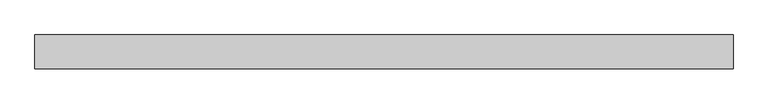
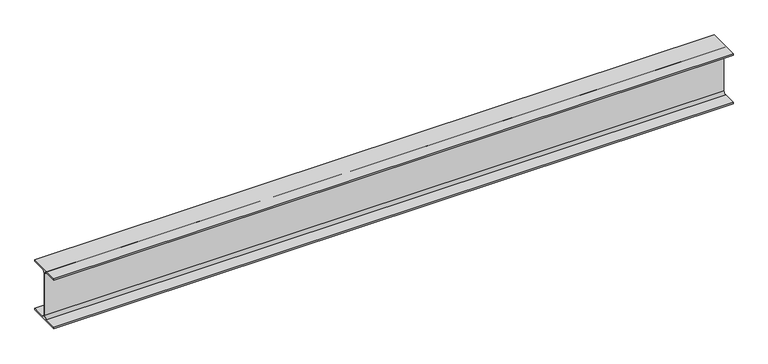
"""IFC4 building model written with IfcOpenShell, lengths in millimetres: beam geometry, 0912_Steel Framing_H-KSD3502 : H_SB_ASB_H-482x300x11x15."""

import ifcopenshell
import ifcopenshell.guid

model = None  # the IFC model being written
_history = None  # IfcOwnerHistory: only IFC2X3 demands one
_inside = {}  # id of a spatial element -> (the spatial element, [elements in it])
_under = {}  # id of a project, library or spatial element -> (it, [spatial elements below it])
_declared = {}  # id of a project -> (the project, [libraries it declares])
_typed = {}  # id of a type object -> (the type object, [elements of that type])
_made_of = {}  # id of a material, layer set ... -> (it, [elements and type objects made of it])


def new_model(schema):
    """Start an empty IFC model of exactly this schema.

    Asked for "IFC4X3", IfcOpenShell would pick the latest addendum, in which some entities
    have other attributes; the version numbers below select the first issue.
    IFC2X3 requires an IfcOwnerHistory on every rooted entity: one is made here for all.
    """
    global model, _history
    if schema == "IFC4X3":
        model = ifcopenshell.file(schema_version=(4, 3, 0, 0))
    else:
        model = ifcopenshell.file(schema=schema)
    _inside.clear()
    _under.clear()
    _declared.clear()
    _typed.clear()
    _made_of.clear()
    _history = None
    if model.schema == "IFC2X3":
        org = make("IfcOrganization", Name="unknown")
        user = make(
            "IfcPersonAndOrganization",
            ThePerson=make("IfcPerson", FamilyName="unknown"),
            TheOrganization=org,
        )
        app = make(
            "IfcApplication",
            ApplicationDeveloper=org,
            Version="unknown",
            ApplicationFullName="unknown",
            ApplicationIdentifier="unknown",
        )
        _history = make(
            "IfcOwnerHistory",
            OwningUser=user,
            OwningApplication=app,
            ChangeAction="ADDED",
            CreationDate=0,
        )
    return model


def make(cls, **values):
    """One entity of the class cls with the attributes given. An attribute that is None is left unset."""
    return model.create_entity(
        cls, **{name: value for name, value in values.items() if value is not None}
    )


def rooted(cls, **values):
    """An entity with a GlobalId (a new one), such as an element, a storey or a relation."""
    return make(cls, GlobalId=ifcopenshell.guid.new(), OwnerHistory=_history, **values)


def si_unit(unit_type, name, prefix=None):
    """IfcSIUnit, for example si_unit("LENGTHUNIT", "METRE", prefix="MILLI")."""
    return make("IfcSIUnit", UnitType=unit_type, Prefix=prefix, Name=name)


def assignment(units):
    """IfcUnitAssignment: the units of a project."""
    return None if units is None else make("IfcUnitAssignment", Units=units)


def point(xyz):
    """IfcCartesianPoint."""
    return None if xyz is None else make("IfcCartesianPoint", Coordinates=xyz)


def direction(xyz):
    """IfcDirection."""
    return None if xyz is None else make("IfcDirection", DirectionRatios=xyz)


def frame(location, z_axis=None, x_axis=None):
    """IfcAxis2Placement3D, a coordinate frame: its origin and axes. An axis left out is left unset."""
    return make(
        "IfcAxis2Placement3D",
        Location=point(location),
        Axis=direction(z_axis),
        RefDirection=direction(x_axis),
    )


def frame_2d(location, x_axis=None):
    """IfcAxis2Placement2D, a coordinate frame in the plane: its origin and x axis."""
    return make(
        "IfcAxis2Placement2D", Location=point(location), RefDirection=direction(x_axis)
    )


def origin():
    """The frame at (0, 0, 0) with its axes left unset."""
    return frame((0.0, 0.0, 0.0))


def place(relative_to, where):
    """IfcLocalPlacement: puts the frame where relative to a parent placement (None: the world)."""
    return make(
        "IfcLocalPlacement", PlacementRelTo=relative_to, RelativePlacement=where
    )


def context(
    kind, dimensions, precision=None, world=None, true_north=None, identifier=None
):
    """IfcGeometricRepresentationContext, for example the 3D "Model" context."""
    return make(
        "IfcGeometricRepresentationContext",
        ContextIdentifier=identifier,
        ContextType=kind,
        CoordinateSpaceDimension=dimensions,
        Precision=precision,
        WorldCoordinateSystem=world,
        TrueNorth=true_north,
    )


def project(units=None, contexts=None):
    """IfcProject with its units and contexts."""
    return rooted(
        "IfcProject",
        Name="project",
        RepresentationContexts=contexts,
        UnitsInContext=assignment(units),
    )


def spatial(cls, under=None, at=None, **own):
    """A site, building, storey or space (cls), placed at a placement, below another one or the project."""
    s = rooted(cls, ObjectPlacement=at, **own)
    if under is not None:
        _under.setdefault(under.id(), (under, []))[1].append(s)
    return s


def polyline(points):
    """IfcPolyline through the points."""
    return make("IfcPolyline", Points=[point(p) for p in points])


def circle_curve(where, radius):
    """IfcCircle in the frame where."""
    return make("IfcCircle", Position=where, Radius=radius)


def trimmed(basis, trim1, trim2, sense, master):
    """IfcTrimmedCurve: the piece of a basis curve between two trims."""
    return make(
        "IfcTrimmedCurve",
        BasisCurve=basis,
        Trim1=trim1,
        Trim2=trim2,
        SenseAgreement=sense,
        MasterRepresentation=master,
    )


def segment(curve, same_sense, transition):
    """IfcCompositeCurveSegment."""
    return make(
        "IfcCompositeCurveSegment",
        Transition=transition,
        SameSense=same_sense,
        ParentCurve=curve,
    )


def composite_curve(segments, self_intersect=None):
    """IfcCompositeCurve: segments joined end to end."""
    return make("IfcCompositeCurve", Segments=segments, SelfIntersect=self_intersect)


def outline(outer, holes=None, kind="AREA"):
    """IfcArbitraryClosedProfileDef: a profile drawn as a closed curve; with holes, ...WithVoids."""
    if holes is None:
        return make("IfcArbitraryClosedProfileDef", ProfileType=kind, OuterCurve=outer)
    return make(
        "IfcArbitraryProfileDefWithVoids",
        ProfileType=kind,
        OuterCurve=outer,
        InnerCurves=holes,
    )


def extrude(swept, where, along, depth):
    """IfcExtrudedAreaSolid: the profile swept, set in the frame where, extruded along a direction by depth."""
    return make(
        "IfcExtrudedAreaSolid",
        SweptArea=swept,
        Position=where,
        ExtrudedDirection=direction(along),
        Depth=depth,
    )


def shape(context_of_items, identifier, shape_type, items):
    """IfcShapeRepresentation: the items that make up one representation, for example the "Body"."""
    return make(
        "IfcShapeRepresentation",
        ContextOfItems=context_of_items,
        RepresentationIdentifier=identifier,
        RepresentationType=shape_type,
        Items=items,
    )


def source(mapping_origin, context_of_items, identifier, shape_type, items):
    """IfcRepresentationMap: a shape defined once, which mapped items show again and again."""
    return make(
        "IfcRepresentationMap",
        MappingOrigin=mapping_origin,
        MappedRepresentation=shape(context_of_items, identifier, shape_type, items),
    )


def transform(
    local_origin,
    x_axis=None,
    y_axis=None,
    z_axis=None,
    scale=None,
    scale2=None,
    scale3=None,
    uniform=True,
):
    """IfcCartesianTransformationOperator3D, or its non-uniform kind. x_axis, y_axis, z_axis: its Axis1, 2, 3."""
    if uniform:
        return make(
            "IfcCartesianTransformationOperator3D",
            Axis1=direction(x_axis),
            Axis2=direction(y_axis),
            LocalOrigin=point(local_origin),
            Scale=scale,
            Axis3=direction(z_axis),
        )
    return make(
        "IfcCartesianTransformationOperator3DnonUniform",
        Axis1=direction(x_axis),
        Axis2=direction(y_axis),
        LocalOrigin=point(local_origin),
        Scale=scale,
        Axis3=direction(z_axis),
        Scale2=scale2,
        Scale3=scale3,
    )


def mapped(mapping_source, mapping_target):
    """IfcMappedItem: shows the shape of a source again, moved by a transform."""
    return make(
        "IfcMappedItem", MappingSource=mapping_source, MappingTarget=mapping_target
    )


def made_of(thing, what):
    """Note that an element or type object is made of a material, layer set ...; save() writes the relation."""
    if what is not None:
        _made_of.setdefault(what.id(), (what, []))[1].append(thing)
    return thing


def element(
    cls,
    number,
    at=None,
    inside=None,
    cuts=None,
    type_object=None,
    material=None,
    context=None,
    identifier="Body",
    shape_type=None,
    held_by="IfcProductDefinitionShape",
    body=None,
    shapes=None,
    **own,
):
    """One element of the class cls, such as IfcWall. Its Tag is "e" and its number.

    at: its placement. inside: the storey or other place that contains it. cuts: it is an
    opening in that element (IfcRelVoidsElement). A single representation is given by context,
    identifier, shape_type and body (its items); several are given by shapes. held_by: the class
    of the entity that holds the representations. save() writes the other relations.
    """
    e = rooted(cls, Tag="e%d" % number, ObjectPlacement=at, **own)
    if body is not None:
        shapes = [shape(context, identifier, shape_type, body)]
    if shapes is not None:
        e.Representation = make(held_by, Representations=shapes)
    if inside is not None:
        _inside.setdefault(inside.id(), (inside, []))[1].append(e)
    if cuts is not None:
        rooted(
            "IfcRelVoidsElement", RelatingBuildingElement=cuts, RelatedOpeningElement=e
        )
    if type_object is not None:
        _typed.setdefault(type_object.id(), (type_object, []))[1].append(e)
    return made_of(e, material)


def aggregate(whole, parts):
    """IfcRelAggregates: a whole, such as a stair, and the parts it consists of."""
    return rooted("IfcRelAggregates", RelatingObject=whole, RelatedObjects=parts)


def save(model, path):
    """Write the relations noted so far, then the file.

    IfcRelAggregates (storeys below a building ...), IfcRelContainedInSpatialStructure (elements
    in a storey), IfcRelDefinesByType, IfcRelAssociatesMaterial and IfcRelDeclares: one each for
    every whole, place, type object, material and project.
    """
    for whole, parts in _under.values():
        aggregate(whole, parts)
    for where, things in _inside.values():
        rooted(
            "IfcRelContainedInSpatialStructure",
            RelatedElements=things,
            RelatingStructure=where,
        )
    for kind, things in _typed.values():
        rooted("IfcRelDefinesByType", RelatedObjects=things, RelatingType=kind)
    for what, things in _made_of.values():
        rooted("IfcRelAssociatesMaterial", RelatedObjects=things, RelatingMaterial=what)
    for by, libraries in _declared.values():
        rooted("IfcRelDeclares", RelatingContext=by, RelatedDefinitions=libraries)
    model.write(path)


def beam_bf8572f3(model_context):
    return source(origin(), model_context, "Body", "SweptSolid", [
        extrude(outline(composite_curve([segment(polyline([(150.0, -226.0), (150.0, -241.0), (-150.0, -241.0), (-150.0, -226.0), (-31.5, -226.0)]), True, "CONTINUOUS"), segment(trimmed(circle_curve(frame_2d((-31.5, -200.0)), 26.0), [point((-31.5, -226.0))], [point((-5.5, -200.0))], True, "CARTESIAN"), True, "CONTINUOUS"), segment(polyline([(-5.5, -200.0), (-5.5, 200.0)]), True, "CONTINUOUS"), segment(trimmed(circle_curve(frame_2d((-31.5, 200.0)), 26.0), [point((-5.5, 200.0))], [point((-31.5, 226.0))], True, "CARTESIAN"), True, "CONTINUOUS"), segment(polyline([(-31.5, 226.0), (-150.0, 226.0), (-150.0, 241.0), (150.0, 241.0), (150.0, 226.0), (31.5, 226.0)]), True, "CONTINUOUS"), segment(trimmed(circle_curve(frame_2d((31.5, 200.0)), 26.0), [point((31.5, 226.0))], [point((5.5, 200.0))], True, "CARTESIAN"), True, "CONTINUOUS"), segment(polyline([(5.5, 200.0), (5.5, -200.0)]), True, "CONTINUOUS"), segment(trimmed(circle_curve(frame_2d((31.5, -200.0)), 26.0), [point((5.5, -200.0))], [point((31.5, -226.0))], True, "CARTESIAN"), True, "CONTINUOUS"), segment(polyline([(31.5, -226.0), (150.0, -226.0)]), True, "CONTINUOUS")], self_intersect=False)), frame((-3087.3, 0.0, 0.0), z_axis=(1.0, 0.0, 0.0), x_axis=(0.0, 1.0, 0.0)), (0.0, 0.0, 1.0), 6174.6),
    ])


if __name__ == "__main__":
    model = new_model("IFC4")
    model_context = context("Model", 3, world=origin())
    ifc_project = project(units=[si_unit("LENGTHUNIT", "METRE", prefix="MILLI")], contexts=[model_context])
    site = spatial("IfcSite", under=ifc_project)
    building = spatial("IfcBuilding", under=site)
    placement = place(None, origin())
    beam_shape = beam_bf8572f3(model_context)
    element("IfcBeam", 1, ObjectType="0912_Steel Framing_H-KSD3502 : H_SB_ASB_H-482x300x11x15", at=placement, inside=building, context=model_context, shape_type="MappedRepresentation", body=[
        mapped(beam_shape, transform((0.0, 0.0, 0.0), x_axis=(1.0, 0.0, 0.0), y_axis=(0.0, 1.0, 0.0), z_axis=(0.0, 0.0, 1.0))),
    ])
    save(model, "model.ifc")

# Revit data of these elements
# Type "0912_Steel Framing_H-KSD3502 : H_SB_ASB_H-482x300x11x15"
#   H_WM Code_1 = "S01AA001-00001 | Main Steel Structure Fabrication Work | Shelter/Building | Heavy Steel - Standard (Weight≥90KG/M) | Material: (   )"
#   H_WM Code_2 = "S03AA027-00001 | Main Steel Structure Erection Work | Shelter/Building | Heavy Steel (Weight≥90KG/M) | Material: (   )"
#   H_WM Code_3 = "S01AA010-00001 | Main Steel Structure Fabrication Work | Shelter/Building | Steel Painting/Coating | for Non-Fireproofed Steel Surface, Surface Preparation, Primer, Second & Final Coat | Material: (   )"
#   H_Q'ty Cal Type Tag = "SB-Q2"
#   Width = 30.0 cm
#   Web Thickness = 1.1 cm
#   Web Fillet = 2.6 cm
#   Warping Constant = 3680000.0 cm⁶
#   W = 0
#   Torsional Moment of Inertia = 88.2192 cm⁴
#   Section Area = 145.5 cm²
#   Plastic Modulus weak axis = 695.0 cm³
#   Plastic Modulus strong axis = 2790.0 cm³
#   Perimeter = 2.10 m²/m
#   Nominal Weight = 114.00 kgf/m
#   Moment of Inertia weak axis = 6760.00 cm⁴
#   Moment of Inertia strong axis = 60400.00 cm⁴
#   Height = 48.2 cm
#   Flange Thickness = 1.5 cm
#   Elastic Modulus weak axis = 451.0 cm³
#   Elastic Modulus strong axis = 2500.0 cm³
#   Centroid Vertical = 24.1 cm
#   Centroid Horizontal = 15.0 cm
#   Ix = 604000000
#   Length [instance default] = 1.5240 m
#   Zx = 2790000
#   b = 0.3000 m
#   h = 0.4820 m
#   r = 0.0260 m
#   s = 0.0110 m
#   t = 0.0150 m
#   A = 0.01455 m²
#   Structural Material [instance default] = Steel, 45-345
#   Assembly Code = ""
# Element 1 (IfcBeam, "0912_Steel Framing_H-KSD3502 : H_SB_ASB_H-482x300x11x15")
#   Structural Material = none
# Materials
#   "Steel, 45-345": class "Metal", colour RGB 189 187 185, transparency 0, Description = "Steel 345 MPa", Cost = 0
